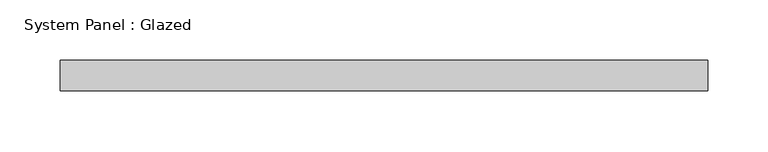
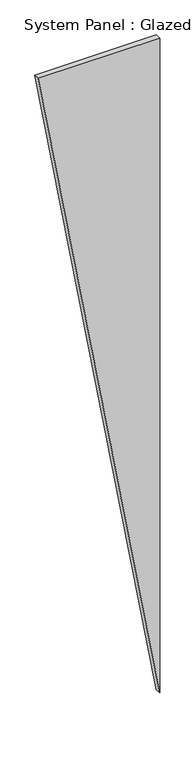
"""IFC4 building model written with IfcOpenShell, lengths in millimetres: plate geometry, System Panel : Glazed."""

from ifc_helpers import new_model, si_unit, frame, origin, place, context, project, spatial, polyline, outline, extrude, source, transform, mapped, element, save


def system_panel_glazed_41c8569a(model_context):
    return source(origin(), model_context, "Body", "SweptSolid", [
        extrude(outline(polyline([(3054.1438606, -268.2393521), (0.0, 268.2393521), (3054.1438606, 268.2393521), (3054.1438606, -268.2393521)])), frame((0.0, -44.45, 0.0), z_axis=(0.0, 1.0, 0.0), x_axis=(0.0, 0.0, 1.0)), (0.0, 0.0, 1.0), 25.4),
    ])


if __name__ == "__main__":
    model = new_model("IFC4")
    model_context = context("Model", 3, world=origin())
    ifc_project = project(units=[si_unit("LENGTHUNIT", "METRE", prefix="MILLI")], contexts=[model_context])
    site = spatial("IfcSite", under=ifc_project)
    building = spatial("IfcBuilding", under=site)
    placement = place(None, origin())
    system_panel_glazed_shape = system_panel_glazed_41c8569a(model_context)
    element("IfcPlate", 1, ObjectType="System Panel : Glazed", at=placement, inside=building, context=model_context, shape_type="MappedRepresentation", body=[
        mapped(system_panel_glazed_shape, transform((0.0, 0.0, 0.0), x_axis=(1.0, 0.0, 0.0), y_axis=(0.0, 1.0, 0.0), z_axis=(0.0, 0.0, 1.0))),
    ])
    save(model, "model.ifc")

# Revit data of these elements
# Type "System Panel : Glazed"
#   Construction Type Id = "GSP4R"
#   Analytic Construction = "1/8 in Pilkington single glazing"
#   Visual Light Transmittance = 0.9
#   Solar Heat Gain Coefficient = 0.86
#   Heat Transfer Coefficient (U) = 1.18115 BTU/(h·ft²·°F)
#   Define Thermal Properties by = 1
# Element 1 (IfcPlate, "System Panel : Glazed")
#   Materials on its faces: "Glass"
# Materials
#   "Glass": class "Glass", colour RGB 0 128 192, transparency 0.75, Description = "Soda Lime Glass", Cost = 0
